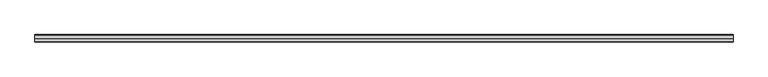
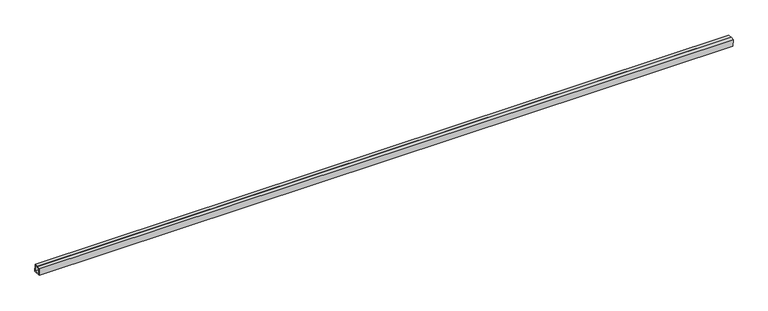
"""IFC4 building model written with IfcOpenShell, lengths in millimetres: proxy geometry, Inner panel:Inner panel:1:Inner panel:1 : Inner panel:Inner panel:300324:2:Inner panel:1:Inner panel:1 : Inner panel:Inner panel:300324:2 : Inner panel:Inner panel:1:Inner panel:1 : Inner panel:Inner panel:300324:300043:41 : Inner panel:Inner panel:1:Inner panel:1 : Inner panel:Inner panel:300324:2:Inner panel:1:Inner panel:1 : Inner panel:Inner panel:300324:2 : Inner panel:Inner panel:1:Inner panel:1 : Inner panel:Inner panel:300324:300043:308120."""

import ifcopenshell
import ifcopenshell.guid

model = None  # the IFC model being written
_history = None  # IfcOwnerHistory: only IFC2X3 demands one
_inside = {}  # id of a spatial element -> (the spatial element, [elements in it])
_under = {}  # id of a project, library or spatial element -> (it, [spatial elements below it])
_declared = {}  # id of a project -> (the project, [libraries it declares])
_typed = {}  # id of a type object -> (the type object, [elements of that type])
_made_of = {}  # id of a material, layer set ... -> (it, [elements and type objects made of it])


def new_model(schema):
    """Start an empty IFC model of exactly this schema.

    Asked for "IFC4X3", IfcOpenShell would pick the latest addendum, in which some entities
    have other attributes; the version numbers below select the first issue.
    IFC2X3 requires an IfcOwnerHistory on every rooted entity: one is made here for all.
    """
    global model, _history
    if schema == "IFC4X3":
        model = ifcopenshell.file(schema_version=(4, 3, 0, 0))
    else:
        model = ifcopenshell.file(schema=schema)
    _inside.clear()
    _under.clear()
    _declared.clear()
    _typed.clear()
    _made_of.clear()
    _history = None
    if model.schema == "IFC2X3":
        org = make("IfcOrganization", Name="unknown")
        user = make(
            "IfcPersonAndOrganization",
            ThePerson=make("IfcPerson", FamilyName="unknown"),
            TheOrganization=org,
        )
        app = make(
            "IfcApplication",
            ApplicationDeveloper=org,
            Version="unknown",
            ApplicationFullName="unknown",
            ApplicationIdentifier="unknown",
        )
        _history = make(
            "IfcOwnerHistory",
            OwningUser=user,
            OwningApplication=app,
            ChangeAction="ADDED",
            CreationDate=0,
        )
    return model


def make(cls, **values):
    """One entity of the class cls with the attributes given. An attribute that is None is left unset."""
    return model.create_entity(
        cls, **{name: value for name, value in values.items() if value is not None}
    )


def rooted(cls, **values):
    """An entity with a GlobalId (a new one), such as an element, a storey or a relation."""
    return make(cls, GlobalId=ifcopenshell.guid.new(), OwnerHistory=_history, **values)


def si_unit(unit_type, name, prefix=None):
    """IfcSIUnit, for example si_unit("LENGTHUNIT", "METRE", prefix="MILLI")."""
    return make("IfcSIUnit", UnitType=unit_type, Prefix=prefix, Name=name)


def assignment(units):
    """IfcUnitAssignment: the units of a project."""
    return None if units is None else make("IfcUnitAssignment", Units=units)


def point(xyz):
    """IfcCartesianPoint."""
    return None if xyz is None else make("IfcCartesianPoint", Coordinates=xyz)


def direction(xyz):
    """IfcDirection."""
    return None if xyz is None else make("IfcDirection", DirectionRatios=xyz)


def frame(location, z_axis=None, x_axis=None):
    """IfcAxis2Placement3D, a coordinate frame: its origin and axes. An axis left out is left unset."""
    return make(
        "IfcAxis2Placement3D",
        Location=point(location),
        Axis=direction(z_axis),
        RefDirection=direction(x_axis),
    )


def origin():
    """The frame at (0, 0, 0) with its axes left unset."""
    return frame((0.0, 0.0, 0.0))


def place(relative_to, where):
    """IfcLocalPlacement: puts the frame where relative to a parent placement (None: the world)."""
    return make(
        "IfcLocalPlacement", PlacementRelTo=relative_to, RelativePlacement=where
    )


def context(
    kind, dimensions, precision=None, world=None, true_north=None, identifier=None
):
    """IfcGeometricRepresentationContext, for example the 3D "Model" context."""
    return make(
        "IfcGeometricRepresentationContext",
        ContextIdentifier=identifier,
        ContextType=kind,
        CoordinateSpaceDimension=dimensions,
        Precision=precision,
        WorldCoordinateSystem=world,
        TrueNorth=true_north,
    )


def project(units=None, contexts=None):
    """IfcProject with its units and contexts."""
    return rooted(
        "IfcProject",
        Name="project",
        RepresentationContexts=contexts,
        UnitsInContext=assignment(units),
    )


def spatial(cls, under=None, at=None, **own):
    """A site, building, storey or space (cls), placed at a placement, below another one or the project."""
    s = rooted(cls, ObjectPlacement=at, **own)
    if under is not None:
        _under.setdefault(under.id(), (under, []))[1].append(s)
    return s


def polyline(points):
    """IfcPolyline through the points."""
    return make("IfcPolyline", Points=[point(p) for p in points])


def outline(outer, holes=None, kind="AREA"):
    """IfcArbitraryClosedProfileDef: a profile drawn as a closed curve; with holes, ...WithVoids."""
    if holes is None:
        return make("IfcArbitraryClosedProfileDef", ProfileType=kind, OuterCurve=outer)
    return make(
        "IfcArbitraryProfileDefWithVoids",
        ProfileType=kind,
        OuterCurve=outer,
        InnerCurves=holes,
    )


def extrude(swept, where, along, depth):
    """IfcExtrudedAreaSolid: the profile swept, set in the frame where, extruded along a direction by depth."""
    return make(
        "IfcExtrudedAreaSolid",
        SweptArea=swept,
        Position=where,
        ExtrudedDirection=direction(along),
        Depth=depth,
    )


def shape(context_of_items, identifier, shape_type, items):
    """IfcShapeRepresentation: the items that make up one representation, for example the "Body"."""
    return make(
        "IfcShapeRepresentation",
        ContextOfItems=context_of_items,
        RepresentationIdentifier=identifier,
        RepresentationType=shape_type,
        Items=items,
    )


def source(mapping_origin, context_of_items, identifier, shape_type, items):
    """IfcRepresentationMap: a shape defined once, which mapped items show again and again."""
    return make(
        "IfcRepresentationMap",
        MappingOrigin=mapping_origin,
        MappedRepresentation=shape(context_of_items, identifier, shape_type, items),
    )


def transform(
    local_origin,
    x_axis=None,
    y_axis=None,
    z_axis=None,
    scale=None,
    scale2=None,
    scale3=None,
    uniform=True,
):
    """IfcCartesianTransformationOperator3D, or its non-uniform kind. x_axis, y_axis, z_axis: its Axis1, 2, 3."""
    if uniform:
        return make(
            "IfcCartesianTransformationOperator3D",
            Axis1=direction(x_axis),
            Axis2=direction(y_axis),
            LocalOrigin=point(local_origin),
            Scale=scale,
            Axis3=direction(z_axis),
        )
    return make(
        "IfcCartesianTransformationOperator3DnonUniform",
        Axis1=direction(x_axis),
        Axis2=direction(y_axis),
        LocalOrigin=point(local_origin),
        Scale=scale,
        Axis3=direction(z_axis),
        Scale2=scale2,
        Scale3=scale3,
    )


def mapped(mapping_source, mapping_target):
    """IfcMappedItem: shows the shape of a source again, moved by a transform."""
    return make(
        "IfcMappedItem", MappingSource=mapping_source, MappingTarget=mapping_target
    )


def made_of(thing, what):
    """Note that an element or type object is made of a material, layer set ...; save() writes the relation."""
    if what is not None:
        _made_of.setdefault(what.id(), (what, []))[1].append(thing)
    return thing


def element(
    cls,
    number,
    at=None,
    inside=None,
    cuts=None,
    type_object=None,
    material=None,
    context=None,
    identifier="Body",
    shape_type=None,
    held_by="IfcProductDefinitionShape",
    body=None,
    shapes=None,
    **own,
):
    """One element of the class cls, such as IfcWall. Its Tag is "e" and its number.

    at: its placement. inside: the storey or other place that contains it. cuts: it is an
    opening in that element (IfcRelVoidsElement). A single representation is given by context,
    identifier, shape_type and body (its items); several are given by shapes. held_by: the class
    of the entity that holds the representations. save() writes the other relations.
    """
    e = rooted(cls, Tag="e%d" % number, ObjectPlacement=at, **own)
    if body is not None:
        shapes = [shape(context, identifier, shape_type, body)]
    if shapes is not None:
        e.Representation = make(held_by, Representations=shapes)
    if inside is not None:
        _inside.setdefault(inside.id(), (inside, []))[1].append(e)
    if cuts is not None:
        rooted(
            "IfcRelVoidsElement", RelatingBuildingElement=cuts, RelatedOpeningElement=e
        )
    if type_object is not None:
        _typed.setdefault(type_object.id(), (type_object, []))[1].append(e)
    return made_of(e, material)


def aggregate(whole, parts):
    """IfcRelAggregates: a whole, such as a stair, and the parts it consists of."""
    return rooted("IfcRelAggregates", RelatingObject=whole, RelatedObjects=parts)


def save(model, path):
    """Write the relations noted so far, then the file.

    IfcRelAggregates (storeys below a building ...), IfcRelContainedInSpatialStructure (elements
    in a storey), IfcRelDefinesByType, IfcRelAssociatesMaterial and IfcRelDeclares: one each for
    every whole, place, type object, material and project.
    """
    for whole, parts in _under.values():
        aggregate(whole, parts)
    for where, things in _inside.values():
        rooted(
            "IfcRelContainedInSpatialStructure",
            RelatedElements=things,
            RelatingStructure=where,
        )
    for kind, things in _typed.values():
        rooted("IfcRelDefinesByType", RelatedObjects=things, RelatingType=kind)
    for what, things in _made_of.values():
        rooted("IfcRelAssociatesMaterial", RelatedObjects=things, RelatingMaterial=what)
    for by, libraries in _declared.values():
        rooted("IfcRelDeclares", RelatingContext=by, RelatedDefinitions=libraries)
    model.write(path)


def generic_models_d78e1118(model_context):
    return source(origin(), model_context, "Body", "SweptSolid", [
        extrude(outline(polyline([(-578476.5317668, 3971.7383355), (-578458.2913437, 3972.4983531), (-578456.7052199, 3934.431383), (-578494.77219, 3932.8452593), (-578496.3583138, 3970.9122294), (-578478.1178906, 3971.672247), (-578478.0187579, 3969.2930614), (-578493.8799954, 3968.6321765), (-578492.4921371, 3935.3235776), (-578459.1835383, 3936.7114359), (-578460.5713966, 3970.0200347), (-578476.4326341, 3969.3591498), (-578476.5317668, 3971.7383355)])), frame((612749.9867239, 0.0, 0.0), z_axis=(1.0, 0.0, 0.0), x_axis=(0.0, 1.0, 0.0)), (0.0, 0.0, 1.0), 3657.6),
    ])


if __name__ == "__main__":
    model = new_model("IFC4")
    model_context = context("Model", 3, world=origin())
    ifc_project = project(units=[si_unit("LENGTHUNIT", "METRE", prefix="MILLI")], contexts=[model_context])
    site = spatial("IfcSite", under=ifc_project)
    building = spatial("IfcBuilding", under=site)
    placement = place(None, origin())
    generic_models_shape = generic_models_d78e1118(model_context)
    element("IfcBuildingElementProxy", 1, Name="Inner panel:Inner panel:1:Inner panel:1 : Inner panel:Inner panel:300324:2:Inner panel:1:Inner panel:1 : Inner panel:Inner panel:300324:2 : Inner panel:Inner panel:1:Inner panel:1 : Inner panel:Inner panel:300324:300043:41 : Inner panel:Inner panel:1:Inner panel:1 : Inner panel:Inner panel:300324:2:Inner panel:1:Inner panel:1 : Inner panel:Inner panel:300324:2 : Inner panel:Inner panel:1:Inner panel:1 : Inner panel:Inner panel:300324:300043:308120", ObjectType="Inner panel:Inner panel:1:Inner panel:1 : Inner panel:Inner panel:300324:2:Inner panel:1:Inner panel:1 : Inner panel:Inner panel:300324:2 : Inner panel:Inner panel:1:Inner panel:1 : Inner panel:Inner panel:300324:300043:41 : Inner panel:Inner panel:1:Inner panel:1 : Inner panel:Inner panel:300324:2:Inner panel:1:Inner panel:1 : Inner panel:Inner panel:300324:2 : Inner panel:Inner panel:1:Inner panel:1 : Inner panel:Inner panel:300324:300043:308120", at=placement, inside=building, context=model_context, shape_type="MappedRepresentation", body=[
        mapped(generic_models_shape, transform((0.0, 0.0, 0.0), x_axis=(1.0, 0.0, 0.0), y_axis=(0.0, 1.0, 0.0), z_axis=(0.0, 0.0, 1.0))),
    ])
    save(model, "model.ifc")

# Revit data of these elements
# Type "Inner panel:Inner panel:1:Inner panel:1 : Inner panel:Inner panel:300324:2:Inner panel:1:Inner panel:1 : Inner panel:Inner panel:300324:2 : Inner panel:Inner panel:1:Inner panel:1 : Inner panel:Inner panel:300324:300043:41 : Inner panel:Inner panel:1:Inner panel:1 : Inner panel:Inner panel:300324:2:Inner panel:1:Inner panel:1 : Inner panel:Inner panel:300324:2 : Inner panel:Inner panel:1:Inner panel:1 : Inner panel:Inner panel:300324:300043:308120"
#   NameOverride = "Inner panel:Inner panel:1:Inner panel:1 : Inner panel:Inner panel:300324:2:Inner panel:1:Inner panel:1 : Inner panel:Inner panel:300324:2 : Inner panel:Inner panel:1:Inner panel:1 : Inner panel:Inner panel:300324:300043:308120"
#   ObjectTypeOverride = "Inner panel:1:Inner panel:1 : Inner panel:Inner panel:300324:2 : Inner panel:Inner panel:1:Inner panel:1 : Inner panel:Inner panel:300324:300043"
#   Reference = "Inner panel"
#   Tag = "308120"
# Element 1 (IfcBuildingElementProxy, "Inner panel:Inner panel:1:Inner panel:1 : Inner panel:Inner panel:300324:2:Inner panel:1:Inner panel:1 : Inner panel:Inner panel:300324:2 : Inner panel:Inner panel:1:Inner panel:1 : Inner panel:Inner panel:300324:300043:41 : Inner panel:Inner panel:1:Inner panel:1 : Inner panel:Inner panel:300324:2:Inner panel:1:Inner panel:1 : Inner panel:Inner panel:300324:2 : Inner panel:Inner panel:1:Inner panel:1 : Inner panel:Inner panel:300324:300043:308120")
#   Materials on its faces: "1 1/2\" X 1 1/2\" SPLIT-SEAM SQUARE TUBING (~24\" CANTILEVER FROM C.L. OF GLULAM)"
# Materials
#   "1 1/2\" X 1 1/2\" SPLIT-SEAM SQUARE TUBING (~24\" CANTILEVER FROM C.L. OF GLULAM)": class "Unassigned", colour RGB 202 201 200, transparency 0, Cost = 0
